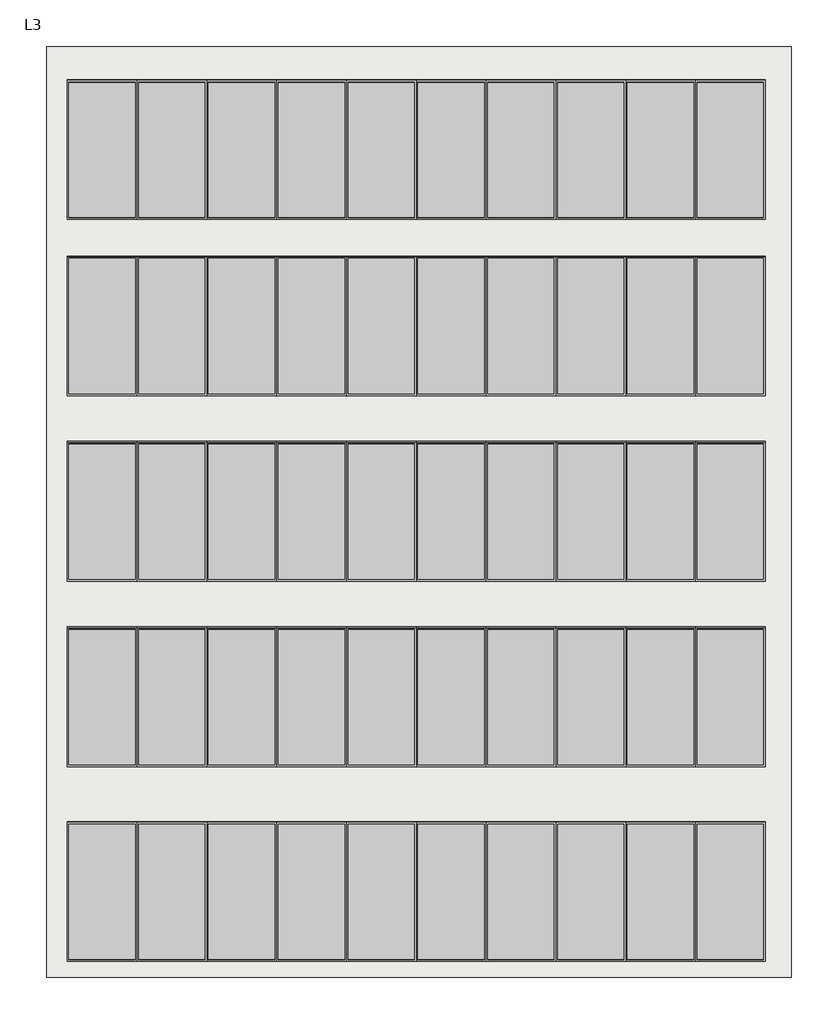
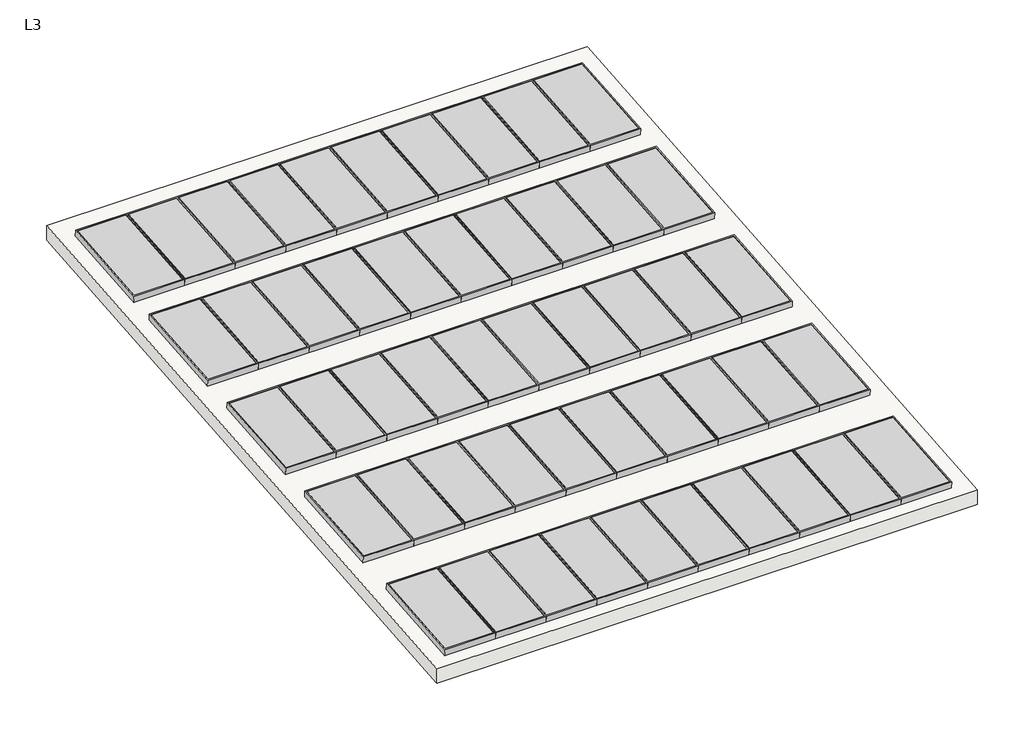
# One storey: 50 proxies, 1 roof.
"""IFC4 building model written with IfcOpenShell, lengths in millimetres."""

import ifcopenshell
import ifcopenshell.guid

model = None  # the IFC model being written
_history = None  # IfcOwnerHistory: only IFC2X3 demands one
_inside = {}  # id of a spatial element -> (the spatial element, [elements in it])
_under = {}  # id of a project, library or spatial element -> (it, [spatial elements below it])
_declared = {}  # id of a project -> (the project, [libraries it declares])
_typed = {}  # id of a type object -> (the type object, [elements of that type])
_made_of = {}  # id of a material, layer set ... -> (it, [elements and type objects made of it])


def new_model(schema):
    """Start an empty IFC model of exactly this schema.

    Asked for "IFC4X3", IfcOpenShell would pick the latest addendum, in which some entities
    have other attributes; the version numbers below select the first issue.
    IFC2X3 requires an IfcOwnerHistory on every rooted entity: one is made here for all.
    """
    global model, _history
    if schema == "IFC4X3":
        model = ifcopenshell.file(schema_version=(4, 3, 0, 0))
    else:
        model = ifcopenshell.file(schema=schema)
    _inside.clear()
    _under.clear()
    _declared.clear()
    _typed.clear()
    _made_of.clear()
    _history = None
    if model.schema == "IFC2X3":
        org = make("IfcOrganization", Name="unknown")
        user = make(
            "IfcPersonAndOrganization",
            ThePerson=make("IfcPerson", FamilyName="unknown"),
            TheOrganization=org,
        )
        app = make(
            "IfcApplication",
            ApplicationDeveloper=org,
            Version="unknown",
            ApplicationFullName="unknown",
            ApplicationIdentifier="unknown",
        )
        _history = make(
            "IfcOwnerHistory",
            OwningUser=user,
            OwningApplication=app,
            ChangeAction="ADDED",
            CreationDate=0,
        )
    return model


def make(cls, **values):
    """One entity of the class cls with the attributes given. An attribute that is None is left unset."""
    return model.create_entity(
        cls, **{name: value for name, value in values.items() if value is not None}
    )


def rooted(cls, **values):
    """An entity with a GlobalId (a new one), such as an element, a storey or a relation."""
    return make(cls, GlobalId=ifcopenshell.guid.new(), OwnerHistory=_history, **values)


def si_unit(unit_type, name, prefix=None):
    """IfcSIUnit, for example si_unit("LENGTHUNIT", "METRE", prefix="MILLI")."""
    return make("IfcSIUnit", UnitType=unit_type, Prefix=prefix, Name=name)


def assignment(units):
    """IfcUnitAssignment: the units of a project."""
    return None if units is None else make("IfcUnitAssignment", Units=units)


def point(xyz):
    """IfcCartesianPoint."""
    return None if xyz is None else make("IfcCartesianPoint", Coordinates=xyz)


def direction(xyz):
    """IfcDirection."""
    return None if xyz is None else make("IfcDirection", DirectionRatios=xyz)


def frame(location, z_axis=None, x_axis=None):
    """IfcAxis2Placement3D, a coordinate frame: its origin and axes. An axis left out is left unset."""
    return make(
        "IfcAxis2Placement3D",
        Location=point(location),
        Axis=direction(z_axis),
        RefDirection=direction(x_axis),
    )


def origin():
    """The frame at (0, 0, 0) with its axes left unset."""
    return frame((0.0, 0.0, 0.0))


def origin_with_axes():
    """The frame at (0, 0, 0) with the z axis (0, 0, 1) and the x axis (1, 0, 0) written out."""
    return frame((0.0, 0.0, 0.0), z_axis=(0.0, 0.0, 1.0), x_axis=(1.0, 0.0, 0.0))


def place(relative_to, where):
    """IfcLocalPlacement: puts the frame where relative to a parent placement (None: the world)."""
    return make(
        "IfcLocalPlacement", PlacementRelTo=relative_to, RelativePlacement=where
    )


def context(
    kind, dimensions, precision=None, world=None, true_north=None, identifier=None
):
    """IfcGeometricRepresentationContext, for example the 3D "Model" context."""
    return make(
        "IfcGeometricRepresentationContext",
        ContextIdentifier=identifier,
        ContextType=kind,
        CoordinateSpaceDimension=dimensions,
        Precision=precision,
        WorldCoordinateSystem=world,
        TrueNorth=true_north,
    )


def project(units=None, contexts=None):
    """IfcProject with its units and contexts."""
    return rooted(
        "IfcProject",
        Name="project",
        RepresentationContexts=contexts,
        UnitsInContext=assignment(units),
    )


def spatial(cls, under=None, at=None, **own):
    """A site, building, storey or space (cls), placed at a placement, below another one or the project."""
    s = rooted(cls, ObjectPlacement=at, **own)
    if under is not None:
        _under.setdefault(under.id(), (under, []))[1].append(s)
    return s


def polyline(points):
    """IfcPolyline through the points."""
    return make("IfcPolyline", Points=[point(p) for p in points])


def outline(outer, holes=None, kind="AREA"):
    """IfcArbitraryClosedProfileDef: a profile drawn as a closed curve; with holes, ...WithVoids."""
    if holes is None:
        return make("IfcArbitraryClosedProfileDef", ProfileType=kind, OuterCurve=outer)
    return make(
        "IfcArbitraryProfileDefWithVoids",
        ProfileType=kind,
        OuterCurve=outer,
        InnerCurves=holes,
    )


def extrude(swept, where, along, depth):
    """IfcExtrudedAreaSolid: the profile swept, set in the frame where, extruded along a direction by depth."""
    return make(
        "IfcExtrudedAreaSolid",
        SweptArea=swept,
        Position=where,
        ExtrudedDirection=direction(along),
        Depth=depth,
    )


def shape(context_of_items, identifier, shape_type, items):
    """IfcShapeRepresentation: the items that make up one representation, for example the "Body"."""
    return make(
        "IfcShapeRepresentation",
        ContextOfItems=context_of_items,
        RepresentationIdentifier=identifier,
        RepresentationType=shape_type,
        Items=items,
    )


def source(mapping_origin, context_of_items, identifier, shape_type, items):
    """IfcRepresentationMap: a shape defined once, which mapped items show again and again."""
    return make(
        "IfcRepresentationMap",
        MappingOrigin=mapping_origin,
        MappedRepresentation=shape(context_of_items, identifier, shape_type, items),
    )


def transform(
    local_origin,
    x_axis=None,
    y_axis=None,
    z_axis=None,
    scale=None,
    scale2=None,
    scale3=None,
    uniform=True,
):
    """IfcCartesianTransformationOperator3D, or its non-uniform kind. x_axis, y_axis, z_axis: its Axis1, 2, 3."""
    if uniform:
        return make(
            "IfcCartesianTransformationOperator3D",
            Axis1=direction(x_axis),
            Axis2=direction(y_axis),
            LocalOrigin=point(local_origin),
            Scale=scale,
            Axis3=direction(z_axis),
        )
    return make(
        "IfcCartesianTransformationOperator3DnonUniform",
        Axis1=direction(x_axis),
        Axis2=direction(y_axis),
        LocalOrigin=point(local_origin),
        Scale=scale,
        Axis3=direction(z_axis),
        Scale2=scale2,
        Scale3=scale3,
    )


def mapped(mapping_source, mapping_target):
    """IfcMappedItem: shows the shape of a source again, moved by a transform."""
    return make(
        "IfcMappedItem", MappingSource=mapping_source, MappingTarget=mapping_target
    )


def made_of(thing, what):
    """Note that an element or type object is made of a material, layer set ...; save() writes the relation."""
    if what is not None:
        _made_of.setdefault(what.id(), (what, []))[1].append(thing)
    return thing


def element(
    cls,
    number,
    at=None,
    inside=None,
    cuts=None,
    type_object=None,
    material=None,
    context=None,
    identifier="Body",
    shape_type=None,
    held_by="IfcProductDefinitionShape",
    body=None,
    shapes=None,
    **own,
):
    """One element of the class cls, such as IfcWall. Its Tag is "e" and its number.

    at: its placement. inside: the storey or other place that contains it. cuts: it is an
    opening in that element (IfcRelVoidsElement). A single representation is given by context,
    identifier, shape_type and body (its items); several are given by shapes. held_by: the class
    of the entity that holds the representations. save() writes the other relations.
    """
    e = rooted(cls, Tag="e%d" % number, ObjectPlacement=at, **own)
    if body is not None:
        shapes = [shape(context, identifier, shape_type, body)]
    if shapes is not None:
        e.Representation = make(held_by, Representations=shapes)
    if inside is not None:
        _inside.setdefault(inside.id(), (inside, []))[1].append(e)
    if cuts is not None:
        rooted(
            "IfcRelVoidsElement", RelatingBuildingElement=cuts, RelatedOpeningElement=e
        )
    if type_object is not None:
        _typed.setdefault(type_object.id(), (type_object, []))[1].append(e)
    return made_of(e, material)


def aggregate(whole, parts):
    """IfcRelAggregates: a whole, such as a stair, and the parts it consists of."""
    return rooted("IfcRelAggregates", RelatingObject=whole, RelatedObjects=parts)


def save(model, path):
    """Write the relations noted so far, then the file.

    IfcRelAggregates (storeys below a building ...), IfcRelContainedInSpatialStructure (elements
    in a storey), IfcRelDefinesByType, IfcRelAssociatesMaterial and IfcRelDeclares: one each for
    every whole, place, type object, material and project.
    """
    for whole, parts in _under.values():
        aggregate(whole, parts)
    for where, things in _inside.values():
        rooted(
            "IfcRelContainedInSpatialStructure",
            RelatedElements=things,
            RelatingStructure=where,
        )
    for kind, things in _typed.values():
        rooted("IfcRelDefinesByType", RelatedObjects=things, RelatingType=kind)
    for what, things in _made_of.values():
        rooted("IfcRelAssociatesMaterial", RelatedObjects=things, RelatingMaterial=what)
    for by, libraries in _declared.values():
        rooted("IfcRelDeclares", RelatingContext=by, RelatedDefinitions=libraries)
    model.write(path)


def m_solar_panel_750_x_1500mm_21fb4d5c(model_context):
    return source(origin(), model_context, "Body", "SweptSolid", [
        extrude(outline(polyline([(32.32, 1500.0), (782.32, 1500.0), (782.32, 0.0), (32.32, 0.0), (32.32, 1500.0)]), holes=[polyline([(763.27, 1480.95), (51.37, 1480.95), (51.37, 19.05), (763.27, 19.05), (763.27, 1480.95)])]), origin_with_axes(), (0.0, 0.0, 1.0), 100.0),
        extrude(outline(polyline([(763.27, 1480.95), (763.27, 19.05), (51.37, 19.05), (51.37, 1480.95), (763.27, 1480.95)])), origin_with_axes(), (0.0, 0.0, 1.0), 93.65),
    ])


model = new_model("IFC4")

# Units and contexts
model_context = context("Model", 3, world=origin())
ifc_project = project(units=[si_unit("LENGTHUNIT", "METRE", prefix="MILLI")], contexts=[model_context])

# Site, building, storey
site = spatial("IfcSite", under=ifc_project)
building = spatial("IfcBuilding", under=site)
storey = spatial("IfcBuildingStorey", under=building, Name="L3", Elevation=6000.0)

# Proxies
placement = place(None, origin())
m_solar_panel_750_x_1500mm_shape = m_solar_panel_750_x_1500mm_21fb4d5c(model_context)
element("IfcBuildingElementProxy", 1, Name="M_Solar Panel : 750 x 1500mm", ObjectType="M_Solar Panel : 750 x 1500mm", at=placement, inside=storey, context=model_context, shape_type="MappedRepresentation", body=[
    mapped(m_solar_panel_750_x_1500mm_shape, transform((-3812.32, 2651.1818746, 6938.9954718), x_axis=(1.0, 0.0, 0.0), y_axis=(0.0, 0.9961946980917455, 0.08715574274765815), z_axis=(0.0, -0.08715574274765815, 0.9961946980917455))),
])
element("IfcBuildingElementProxy", 2, Name="M_Solar Panel : 750 x 1500mm", ObjectType="M_Solar Panel : 750 x 1500mm", at=placement, inside=storey, context=model_context, shape_type="MappedRepresentation", body=[
    mapped(m_solar_panel_750_x_1500mm_shape, transform((-3062.32, 2651.1818746, 6938.9954718), x_axis=(1.0, 0.0, 0.0), y_axis=(0.0, 0.9961946980917455, 0.08715574274765815), z_axis=(0.0, -0.08715574274765815, 0.9961946980917455))),
])
element("IfcBuildingElementProxy", 3, Name="M_Solar Panel : 750 x 1500mm", ObjectType="M_Solar Panel : 750 x 1500mm", at=placement, inside=storey, context=model_context, shape_type="MappedRepresentation", body=[
    mapped(m_solar_panel_750_x_1500mm_shape, transform((-2312.32, 2651.1818746, 6938.9954718), x_axis=(1.0, 0.0, 0.0), y_axis=(0.0, 0.9961946980917455, 0.08715574274765815), z_axis=(0.0, -0.08715574274765815, 0.9961946980917455))),
])
element("IfcBuildingElementProxy", 4, Name="M_Solar Panel : 750 x 1500mm", ObjectType="M_Solar Panel : 750 x 1500mm", at=placement, inside=storey, context=model_context, shape_type="MappedRepresentation", body=[
    mapped(m_solar_panel_750_x_1500mm_shape, transform((-1562.32, 2651.1818746, 6938.9954718), x_axis=(1.0, 0.0, 0.0), y_axis=(0.0, 0.9961946980917455, 0.08715574274765815), z_axis=(0.0, -0.08715574274765815, 0.9961946980917455))),
])
element("IfcBuildingElementProxy", 5, Name="M_Solar Panel : 750 x 1500mm", ObjectType="M_Solar Panel : 750 x 1500mm", at=placement, inside=storey, context=model_context, shape_type="MappedRepresentation", body=[
    mapped(m_solar_panel_750_x_1500mm_shape, transform((-812.32, 2651.1818746, 6938.9954718), x_axis=(1.0, 0.0, 0.0), y_axis=(0.0, 0.9961946980917455, 0.08715574274765815), z_axis=(0.0, -0.08715574274765815, 0.9961946980917455))),
])
element("IfcBuildingElementProxy", 6, Name="M_Solar Panel : 750 x 1500mm", ObjectType="M_Solar Panel : 750 x 1500mm", at=placement, inside=storey, context=model_context, shape_type="MappedRepresentation", body=[
    mapped(m_solar_panel_750_x_1500mm_shape, transform((-62.32, 2651.1818746, 6938.9954718), x_axis=(1.0, 0.0, 0.0), y_axis=(0.0, 0.9961946980917455, 0.08715574274765815), z_axis=(0.0, -0.08715574274765815, 0.9961946980917455))),
])
element("IfcBuildingElementProxy", 7, Name="M_Solar Panel : 750 x 1500mm", ObjectType="M_Solar Panel : 750 x 1500mm", at=placement, inside=storey, context=model_context, shape_type="MappedRepresentation", body=[
    mapped(m_solar_panel_750_x_1500mm_shape, transform((687.68, 2651.1818746, 6938.9954718), x_axis=(1.0, 0.0, 0.0), y_axis=(0.0, 0.9961946980917455, 0.08715574274765815), z_axis=(0.0, -0.08715574274765815, 0.9961946980917455))),
])
element("IfcBuildingElementProxy", 8, Name="M_Solar Panel : 750 x 1500mm", ObjectType="M_Solar Panel : 750 x 1500mm", at=placement, inside=storey, context=model_context, shape_type="MappedRepresentation", body=[
    mapped(m_solar_panel_750_x_1500mm_shape, transform((1437.68, 2651.1818746, 6938.9954718), x_axis=(1.0, 0.0, 0.0), y_axis=(0.0, 0.9961946980917455, 0.08715574274765815), z_axis=(0.0, -0.08715574274765815, 0.9961946980917455))),
])
element("IfcBuildingElementProxy", 9, Name="M_Solar Panel : 750 x 1500mm", ObjectType="M_Solar Panel : 750 x 1500mm", at=placement, inside=storey, context=model_context, shape_type="MappedRepresentation", body=[
    mapped(m_solar_panel_750_x_1500mm_shape, transform((2187.68, 2651.1818746, 6938.9954718), x_axis=(1.0, 0.0, 0.0), y_axis=(0.0, 0.9961946980917455, 0.08715574274765815), z_axis=(0.0, -0.08715574274765815, 0.9961946980917455))),
])
element("IfcBuildingElementProxy", 10, Name="M_Solar Panel : 750 x 1500mm", ObjectType="M_Solar Panel : 750 x 1500mm", at=placement, inside=storey, context=model_context, shape_type="MappedRepresentation", body=[
    mapped(m_solar_panel_750_x_1500mm_shape, transform((2937.68, 2651.1818746, 6938.9954718), x_axis=(1.0, 0.0, 0.0), y_axis=(0.0, 0.9961946980917455, 0.08715574274765815), z_axis=(0.0, -0.08715574274765815, 0.9961946980917455))),
])
element("IfcBuildingElementProxy", 11, Name="M_Solar Panel : 750 x 1500mm", ObjectType="M_Solar Panel : 750 x 1500mm", at=placement, inside=storey, context=model_context, shape_type="MappedRepresentation", body=[
    mapped(m_solar_panel_750_x_1500mm_shape, transform((-3812.32, 758.4119482, 6773.3995606), x_axis=(1.0, 0.0, 0.0), y_axis=(0.0, 0.9961946980917455, 0.08715574274765815), z_axis=(0.0, -0.08715574274765815, 0.9961946980917455))),
])
element("IfcBuildingElementProxy", 12, Name="M_Solar Panel : 750 x 1500mm", ObjectType="M_Solar Panel : 750 x 1500mm", at=placement, inside=storey, context=model_context, shape_type="MappedRepresentation", body=[
    mapped(m_solar_panel_750_x_1500mm_shape, transform((-3062.32, 758.4119482, 6773.3995606), x_axis=(1.0, 0.0, 0.0), y_axis=(0.0, 0.9961946980917455, 0.08715574274765815), z_axis=(0.0, -0.08715574274765815, 0.9961946980917455))),
])
element("IfcBuildingElementProxy", 13, Name="M_Solar Panel : 750 x 1500mm", ObjectType="M_Solar Panel : 750 x 1500mm", at=placement, inside=storey, context=model_context, shape_type="MappedRepresentation", body=[
    mapped(m_solar_panel_750_x_1500mm_shape, transform((-2312.32, 758.4119482, 6773.3995606), x_axis=(1.0, 0.0, 0.0), y_axis=(0.0, 0.9961946980917455, 0.08715574274765815), z_axis=(0.0, -0.08715574274765815, 0.9961946980917455))),
])
element("IfcBuildingElementProxy", 14, Name="M_Solar Panel : 750 x 1500mm", ObjectType="M_Solar Panel : 750 x 1500mm", at=placement, inside=storey, context=model_context, shape_type="MappedRepresentation", body=[
    mapped(m_solar_panel_750_x_1500mm_shape, transform((-1562.32, 758.4119482, 6773.3995606), x_axis=(1.0, 0.0, 0.0), y_axis=(0.0, 0.9961946980917455, 0.08715574274765815), z_axis=(0.0, -0.08715574274765815, 0.9961946980917455))),
])
element("IfcBuildingElementProxy", 15, Name="M_Solar Panel : 750 x 1500mm", ObjectType="M_Solar Panel : 750 x 1500mm", at=placement, inside=storey, context=model_context, shape_type="MappedRepresentation", body=[
    mapped(m_solar_panel_750_x_1500mm_shape, transform((-812.32, 758.4119482, 6773.3995606), x_axis=(1.0, 0.0, 0.0), y_axis=(0.0, 0.9961946980917455, 0.08715574274765815), z_axis=(0.0, -0.08715574274765815, 0.9961946980917455))),
])
element("IfcBuildingElementProxy", 16, Name="M_Solar Panel : 750 x 1500mm", ObjectType="M_Solar Panel : 750 x 1500mm", at=placement, inside=storey, context=model_context, shape_type="MappedRepresentation", body=[
    mapped(m_solar_panel_750_x_1500mm_shape, transform((-62.32, 758.4119482, 6773.3995606), x_axis=(1.0, 0.0, 0.0), y_axis=(0.0, 0.9961946980917455, 0.08715574274765815), z_axis=(0.0, -0.08715574274765815, 0.9961946980917455))),
])
element("IfcBuildingElementProxy", 17, Name="M_Solar Panel : 750 x 1500mm", ObjectType="M_Solar Panel : 750 x 1500mm", at=placement, inside=storey, context=model_context, shape_type="MappedRepresentation", body=[
    mapped(m_solar_panel_750_x_1500mm_shape, transform((687.68, 758.4119482, 6773.3995606), x_axis=(1.0, 0.0, 0.0), y_axis=(0.0, 0.9961946980917455, 0.08715574274765815), z_axis=(0.0, -0.08715574274765815, 0.9961946980917455))),
])
element("IfcBuildingElementProxy", 18, Name="M_Solar Panel : 750 x 1500mm", ObjectType="M_Solar Panel : 750 x 1500mm", at=placement, inside=storey, context=model_context, shape_type="MappedRepresentation", body=[
    mapped(m_solar_panel_750_x_1500mm_shape, transform((1437.68, 758.4119482, 6773.3995606), x_axis=(1.0, 0.0, 0.0), y_axis=(0.0, 0.9961946980917455, 0.08715574274765815), z_axis=(0.0, -0.08715574274765815, 0.9961946980917455))),
])
element("IfcBuildingElementProxy", 19, Name="M_Solar Panel : 750 x 1500mm", ObjectType="M_Solar Panel : 750 x 1500mm", at=placement, inside=storey, context=model_context, shape_type="MappedRepresentation", body=[
    mapped(m_solar_panel_750_x_1500mm_shape, transform((2187.68, 758.4119482, 6773.3995606), x_axis=(1.0, 0.0, 0.0), y_axis=(0.0, 0.9961946980917455, 0.08715574274765815), z_axis=(0.0, -0.08715574274765815, 0.9961946980917455))),
])
element("IfcBuildingElementProxy", 20, Name="M_Solar Panel : 750 x 1500mm", ObjectType="M_Solar Panel : 750 x 1500mm", at=placement, inside=storey, context=model_context, shape_type="MappedRepresentation", body=[
    mapped(m_solar_panel_750_x_1500mm_shape, transform((2937.68, 758.4119482, 6773.3995606), x_axis=(1.0, 0.0, 0.0), y_axis=(0.0, 0.9961946980917455, 0.08715574274765815), z_axis=(0.0, -0.08715574274765815, 0.9961946980917455))),
])
element("IfcBuildingElementProxy", 21, Name="M_Solar Panel : 750 x 1500mm", ObjectType="M_Solar Panel : 750 x 1500mm", at=placement, inside=storey, context=model_context, shape_type="MappedRepresentation", body=[
    mapped(m_solar_panel_750_x_1500mm_shape, transform((-3812.32, -1233.9774479, 6599.0880751), x_axis=(1.0, 0.0, 0.0), y_axis=(0.0, 0.9961946980917455, 0.08715574274765815), z_axis=(0.0, -0.08715574274765815, 0.9961946980917455))),
])
element("IfcBuildingElementProxy", 22, Name="M_Solar Panel : 750 x 1500mm", ObjectType="M_Solar Panel : 750 x 1500mm", at=placement, inside=storey, context=model_context, shape_type="MappedRepresentation", body=[
    mapped(m_solar_panel_750_x_1500mm_shape, transform((-3062.32, -1233.9774479, 6599.0880751), x_axis=(1.0, 0.0, 0.0), y_axis=(0.0, 0.9961946980917455, 0.08715574274765815), z_axis=(0.0, -0.08715574274765815, 0.9961946980917455))),
])
element("IfcBuildingElementProxy", 23, Name="M_Solar Panel : 750 x 1500mm", ObjectType="M_Solar Panel : 750 x 1500mm", at=placement, inside=storey, context=model_context, shape_type="MappedRepresentation", body=[
    mapped(m_solar_panel_750_x_1500mm_shape, transform((-2312.32, -1233.9774479, 6599.0880751), x_axis=(1.0, 0.0, 0.0), y_axis=(0.0, 0.9961946980917455, 0.08715574274765815), z_axis=(0.0, -0.08715574274765815, 0.9961946980917455))),
])
element("IfcBuildingElementProxy", 24, Name="M_Solar Panel : 750 x 1500mm", ObjectType="M_Solar Panel : 750 x 1500mm", at=placement, inside=storey, context=model_context, shape_type="MappedRepresentation", body=[
    mapped(m_solar_panel_750_x_1500mm_shape, transform((-1562.32, -1233.9774479, 6599.0880751), x_axis=(1.0, 0.0, 0.0), y_axis=(0.0, 0.9961946980917455, 0.08715574274765815), z_axis=(0.0, -0.08715574274765815, 0.9961946980917455))),
])
element("IfcBuildingElementProxy", 25, Name="M_Solar Panel : 750 x 1500mm", ObjectType="M_Solar Panel : 750 x 1500mm", at=placement, inside=storey, context=model_context, shape_type="MappedRepresentation", body=[
    mapped(m_solar_panel_750_x_1500mm_shape, transform((-812.32, -1233.9774479, 6599.0880751), x_axis=(1.0, 0.0, 0.0), y_axis=(0.0, 0.9961946980917455, 0.08715574274765815), z_axis=(0.0, -0.08715574274765815, 0.9961946980917455))),
])
element("IfcBuildingElementProxy", 26, Name="M_Solar Panel : 750 x 1500mm", ObjectType="M_Solar Panel : 750 x 1500mm", at=placement, inside=storey, context=model_context, shape_type="MappedRepresentation", body=[
    mapped(m_solar_panel_750_x_1500mm_shape, transform((-62.32, -1233.9774479, 6599.0880751), x_axis=(1.0, 0.0, 0.0), y_axis=(0.0, 0.9961946980917455, 0.08715574274765815), z_axis=(0.0, -0.08715574274765815, 0.9961946980917455))),
])
element("IfcBuildingElementProxy", 27, Name="M_Solar Panel : 750 x 1500mm", ObjectType="M_Solar Panel : 750 x 1500mm", at=placement, inside=storey, context=model_context, shape_type="MappedRepresentation", body=[
    mapped(m_solar_panel_750_x_1500mm_shape, transform((687.68, -1233.9774479, 6599.0880751), x_axis=(1.0, 0.0, 0.0), y_axis=(0.0, 0.9961946980917455, 0.08715574274765815), z_axis=(0.0, -0.08715574274765815, 0.9961946980917455))),
])
element("IfcBuildingElementProxy", 28, Name="M_Solar Panel : 750 x 1500mm", ObjectType="M_Solar Panel : 750 x 1500mm", at=placement, inside=storey, context=model_context, shape_type="MappedRepresentation", body=[
    mapped(m_solar_panel_750_x_1500mm_shape, transform((1437.68, -1233.9774479, 6599.0880751), x_axis=(1.0, 0.0, 0.0), y_axis=(0.0, 0.9961946980917455, 0.08715574274765815), z_axis=(0.0, -0.08715574274765815, 0.9961946980917455))),
])
element("IfcBuildingElementProxy", 29, Name="M_Solar Panel : 750 x 1500mm", ObjectType="M_Solar Panel : 750 x 1500mm", at=placement, inside=storey, context=model_context, shape_type="MappedRepresentation", body=[
    mapped(m_solar_panel_750_x_1500mm_shape, transform((2187.68, -1233.9774479, 6599.0880751), x_axis=(1.0, 0.0, 0.0), y_axis=(0.0, 0.9961946980917455, 0.08715574274765815), z_axis=(0.0, -0.08715574274765815, 0.9961946980917455))),
])
element("IfcBuildingElementProxy", 30, Name="M_Solar Panel : 750 x 1500mm", ObjectType="M_Solar Panel : 750 x 1500mm", at=placement, inside=storey, context=model_context, shape_type="MappedRepresentation", body=[
    mapped(m_solar_panel_750_x_1500mm_shape, transform((2937.68, -1233.9774479, 6599.0880751), x_axis=(1.0, 0.0, 0.0), y_axis=(0.0, 0.9961946980917455, 0.08715574274765815), z_axis=(0.0, -0.08715574274765815, 0.9961946980917455))),
])
element("IfcBuildingElementProxy", 31, Name="M_Solar Panel : 750 x 1500mm", ObjectType="M_Solar Panel : 750 x 1500mm", at=placement, inside=storey, context=model_context, shape_type="MappedRepresentation", body=[
    mapped(m_solar_panel_750_x_1500mm_shape, transform((-3812.32, -3226.3668441, 6424.7765896), x_axis=(1.0, 0.0, 0.0), y_axis=(0.0, 0.9961946980917455, 0.08715574274765815), z_axis=(0.0, -0.08715574274765815, 0.9961946980917455))),
])
element("IfcBuildingElementProxy", 32, Name="M_Solar Panel : 750 x 1500mm", ObjectType="M_Solar Panel : 750 x 1500mm", at=placement, inside=storey, context=model_context, shape_type="MappedRepresentation", body=[
    mapped(m_solar_panel_750_x_1500mm_shape, transform((-3062.32, -3226.3668441, 6424.7765896), x_axis=(1.0, 0.0, 0.0), y_axis=(0.0, 0.9961946980917455, 0.08715574274765815), z_axis=(0.0, -0.08715574274765815, 0.9961946980917455))),
])
element("IfcBuildingElementProxy", 33, Name="M_Solar Panel : 750 x 1500mm", ObjectType="M_Solar Panel : 750 x 1500mm", at=placement, inside=storey, context=model_context, shape_type="MappedRepresentation", body=[
    mapped(m_solar_panel_750_x_1500mm_shape, transform((-2312.32, -3226.3668441, 6424.7765896), x_axis=(1.0, 0.0, 0.0), y_axis=(0.0, 0.9961946980917455, 0.08715574274765815), z_axis=(0.0, -0.08715574274765815, 0.9961946980917455))),
])
element("IfcBuildingElementProxy", 34, Name="M_Solar Panel : 750 x 1500mm", ObjectType="M_Solar Panel : 750 x 1500mm", at=placement, inside=storey, context=model_context, shape_type="MappedRepresentation", body=[
    mapped(m_solar_panel_750_x_1500mm_shape, transform((-1562.32, -3226.3668441, 6424.7765896), x_axis=(1.0, 0.0, 0.0), y_axis=(0.0, 0.9961946980917455, 0.08715574274765815), z_axis=(0.0, -0.08715574274765815, 0.9961946980917455))),
])
element("IfcBuildingElementProxy", 35, Name="M_Solar Panel : 750 x 1500mm", ObjectType="M_Solar Panel : 750 x 1500mm", at=placement, inside=storey, context=model_context, shape_type="MappedRepresentation", body=[
    mapped(m_solar_panel_750_x_1500mm_shape, transform((-812.32, -3226.3668441, 6424.7765896), x_axis=(1.0, 0.0, 0.0), y_axis=(0.0, 0.9961946980917455, 0.08715574274765815), z_axis=(0.0, -0.08715574274765815, 0.9961946980917455))),
])
element("IfcBuildingElementProxy", 36, Name="M_Solar Panel : 750 x 1500mm", ObjectType="M_Solar Panel : 750 x 1500mm", at=placement, inside=storey, context=model_context, shape_type="MappedRepresentation", body=[
    mapped(m_solar_panel_750_x_1500mm_shape, transform((-62.32, -3226.3668441, 6424.7765896), x_axis=(1.0, 0.0, 0.0), y_axis=(0.0, 0.9961946980917455, 0.08715574274765815), z_axis=(0.0, -0.08715574274765815, 0.9961946980917455))),
])
element("IfcBuildingElementProxy", 37, Name="M_Solar Panel : 750 x 1500mm", ObjectType="M_Solar Panel : 750 x 1500mm", at=placement, inside=storey, context=model_context, shape_type="MappedRepresentation", body=[
    mapped(m_solar_panel_750_x_1500mm_shape, transform((687.68, -3226.3668441, 6424.7765896), x_axis=(1.0, 0.0, 0.0), y_axis=(0.0, 0.9961946980917455, 0.08715574274765815), z_axis=(0.0, -0.08715574274765815, 0.9961946980917455))),
])
element("IfcBuildingElementProxy", 38, Name="M_Solar Panel : 750 x 1500mm", ObjectType="M_Solar Panel : 750 x 1500mm", at=placement, inside=storey, context=model_context, shape_type="MappedRepresentation", body=[
    mapped(m_solar_panel_750_x_1500mm_shape, transform((1437.68, -3226.3668441, 6424.7765896), x_axis=(1.0, 0.0, 0.0), y_axis=(0.0, 0.9961946980917455, 0.08715574274765815), z_axis=(0.0, -0.08715574274765815, 0.9961946980917455))),
])
element("IfcBuildingElementProxy", 39, Name="M_Solar Panel : 750 x 1500mm", ObjectType="M_Solar Panel : 750 x 1500mm", at=placement, inside=storey, context=model_context, shape_type="MappedRepresentation", body=[
    mapped(m_solar_panel_750_x_1500mm_shape, transform((2187.68, -3226.3668441, 6424.7765896), x_axis=(1.0, 0.0, 0.0), y_axis=(0.0, 0.9961946980917455, 0.08715574274765815), z_axis=(0.0, -0.08715574274765815, 0.9961946980917455))),
])
element("IfcBuildingElementProxy", 40, Name="M_Solar Panel : 750 x 1500mm", ObjectType="M_Solar Panel : 750 x 1500mm", at=placement, inside=storey, context=model_context, shape_type="MappedRepresentation", body=[
    mapped(m_solar_panel_750_x_1500mm_shape, transform((2937.68, -3226.3668441, 6424.7765896), x_axis=(1.0, 0.0, 0.0), y_axis=(0.0, 0.9961946980917455, 0.08715574274765815), z_axis=(0.0, -0.08715574274765815, 0.9961946980917455))),
])
element("IfcBuildingElementProxy", 41, Name="M_Solar Panel : 750 x 1500mm", ObjectType="M_Solar Panel : 750 x 1500mm", at=placement, inside=storey, context=model_context, shape_type="MappedRepresentation", body=[
    mapped(m_solar_panel_750_x_1500mm_shape, transform((-3812.32, -5318.3757101, 6241.7495298), x_axis=(1.0, 0.0, 0.0), y_axis=(0.0, 0.9961946980917455, 0.08715574274765815), z_axis=(0.0, -0.08715574274765815, 0.9961946980917455))),
])
element("IfcBuildingElementProxy", 42, Name="M_Solar Panel : 750 x 1500mm", ObjectType="M_Solar Panel : 750 x 1500mm", at=placement, inside=storey, context=model_context, shape_type="MappedRepresentation", body=[
    mapped(m_solar_panel_750_x_1500mm_shape, transform((-3062.32, -5318.3757101, 6241.7495298), x_axis=(1.0, 0.0, 0.0), y_axis=(0.0, 0.9961946980917455, 0.08715574274765815), z_axis=(0.0, -0.08715574274765815, 0.9961946980917455))),
])
element("IfcBuildingElementProxy", 43, Name="M_Solar Panel : 750 x 1500mm", ObjectType="M_Solar Panel : 750 x 1500mm", at=placement, inside=storey, context=model_context, shape_type="MappedRepresentation", body=[
    mapped(m_solar_panel_750_x_1500mm_shape, transform((-2312.32, -5318.3757101, 6241.7495298), x_axis=(1.0, 0.0, 0.0), y_axis=(0.0, 0.9961946980917455, 0.08715574274765815), z_axis=(0.0, -0.08715574274765815, 0.9961946980917455))),
])
element("IfcBuildingElementProxy", 44, Name="M_Solar Panel : 750 x 1500mm", ObjectType="M_Solar Panel : 750 x 1500mm", at=placement, inside=storey, context=model_context, shape_type="MappedRepresentation", body=[
    mapped(m_solar_panel_750_x_1500mm_shape, transform((-1562.32, -5318.3757101, 6241.7495298), x_axis=(1.0, 0.0, 0.0), y_axis=(0.0, 0.9961946980917455, 0.08715574274765815), z_axis=(0.0, -0.08715574274765815, 0.9961946980917455))),
])
element("IfcBuildingElementProxy", 45, Name="M_Solar Panel : 750 x 1500mm", ObjectType="M_Solar Panel : 750 x 1500mm", at=placement, inside=storey, context=model_context, shape_type="MappedRepresentation", body=[
    mapped(m_solar_panel_750_x_1500mm_shape, transform((-812.32, -5318.3757101, 6241.7495298), x_axis=(1.0, 0.0, 0.0), y_axis=(0.0, 0.9961946980917455, 0.08715574274765815), z_axis=(0.0, -0.08715574274765815, 0.9961946980917455))),
])
element("IfcBuildingElementProxy", 46, Name="M_Solar Panel : 750 x 1500mm", ObjectType="M_Solar Panel : 750 x 1500mm", at=placement, inside=storey, context=model_context, shape_type="MappedRepresentation", body=[
    mapped(m_solar_panel_750_x_1500mm_shape, transform((-62.32, -5318.3757101, 6241.7495298), x_axis=(1.0, 0.0, 0.0), y_axis=(0.0, 0.9961946980917455, 0.08715574274765815), z_axis=(0.0, -0.08715574274765815, 0.9961946980917455))),
])
element("IfcBuildingElementProxy", 47, Name="M_Solar Panel : 750 x 1500mm", ObjectType="M_Solar Panel : 750 x 1500mm", at=placement, inside=storey, context=model_context, shape_type="MappedRepresentation", body=[
    mapped(m_solar_panel_750_x_1500mm_shape, transform((687.68, -5318.3757101, 6241.7495298), x_axis=(1.0, 0.0, 0.0), y_axis=(0.0, 0.9961946980917455, 0.08715574274765815), z_axis=(0.0, -0.08715574274765815, 0.9961946980917455))),
])
element("IfcBuildingElementProxy", 48, Name="M_Solar Panel : 750 x 1500mm", ObjectType="M_Solar Panel : 750 x 1500mm", at=placement, inside=storey, context=model_context, shape_type="MappedRepresentation", body=[
    mapped(m_solar_panel_750_x_1500mm_shape, transform((1437.68, -5318.3757101, 6241.7495298), x_axis=(1.0, 0.0, 0.0), y_axis=(0.0, 0.9961946980917455, 0.08715574274765815), z_axis=(0.0, -0.08715574274765815, 0.9961946980917455))),
])
element("IfcBuildingElementProxy", 49, Name="M_Solar Panel : 750 x 1500mm", ObjectType="M_Solar Panel : 750 x 1500mm", at=placement, inside=storey, context=model_context, shape_type="MappedRepresentation", body=[
    mapped(m_solar_panel_750_x_1500mm_shape, transform((2187.68, -5318.3757101, 6241.7495298), x_axis=(1.0, 0.0, 0.0), y_axis=(0.0, 0.9961946980917455, 0.08715574274765815), z_axis=(0.0, -0.08715574274765815, 0.9961946980917455))),
])
element("IfcBuildingElementProxy", 50, Name="M_Solar Panel : 750 x 1500mm", ObjectType="M_Solar Panel : 750 x 1500mm", at=placement, inside=storey, context=model_context, shape_type="MappedRepresentation", body=[
    mapped(m_solar_panel_750_x_1500mm_shape, transform((2937.68, -5318.3757101, 6241.7495298), x_axis=(1.0, 0.0, 0.0), y_axis=(0.0, 0.9961946980917455, 0.08715574274765815), z_axis=(0.0, -0.08715574274765815, 0.9961946980917455))),
])

# Roof
element("IfcRoof", 51, ObjectType="Genérico - 225 mm", at=placement, inside=storey, context=model_context, shape_type="SweptSolid", body=[
    extrude(outline(polyline([(-5500.0, 6225.8594634), (4500.0, 7100.7460987), (4500.0, 6874.8866353), (-5500.0, 6000.0), (-5500.0, 6225.8594634)])), frame((-4000.0, 0.0, 0.0), z_axis=(1.0, 0.0, 0.0), x_axis=(0.0, 1.0, 0.0)), (0.0, 0.0, 1.0), 8000.0),
])

save(model, "model.ifc")

# Revit data of these elements
# Type "M_Solar Panel : 750 x 1500mm"
#   Width = 0.75 m
#   Length = 1.5 m
#   Depth = 0.1 m
#   Default Elevation = 1.2 m
# Type "Genérico - 225 mm"
#   Description = "Cubierta genérica (material por categoría), grosor de 225 mm"
#   Type Mark = "G01"
#   Layers, outside or top first: 0.225 m no material (function 1)
# Elements 1, 2, 3, 4, 5, 6, 7, 8, 9, 10, 11, 12, 13, 14, 15, 16, 17, 18, 19, 20, 21, 22, 23, 24, 25, 26, 27, 28, 29, 30, 31, 32, 33, 34, 35, 36, 37, 38, 39, 40, 41, 42, 43, 44, 45, 46, 47, 48, 49, 50 (IfcBuildingElementProxy, "M_Solar Panel : 750 x 1500mm")
#   Phase Created = Nueva construcción
#   Materials on its faces: "Metal Trim", "Metal - Aluminum (2)"
# Element 51 (IfcRoof, "Genérico - 225 mm")
#   built-in parameter 1001705 = 23.2964 (stored number, unit not read)
#   built-in parameter 1001710 = 33615
#   Phase Created = Nueva construcción
#   Materials on its faces: "Cubierta por defecto"
# Materials
#   "Metal Trim": class "Metal", colour RGB 247 247 247, transparency 0
#   "Metal - Aluminum (2)": class "Metal", colour RGB 247 247 247, transparency 0
#   "Cubierta por defecto": class "Varios", colour RGB 0 64 0, transparency 0, Cost = 0
